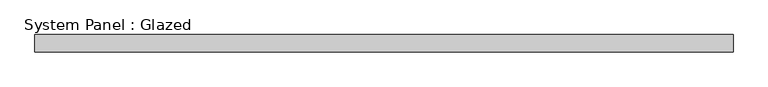
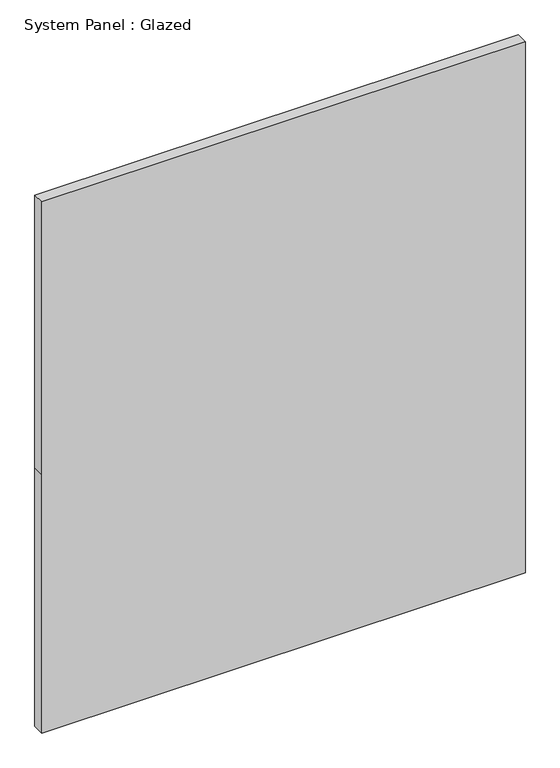
"""IFC4 building model written with IfcOpenShell, lengths in millimetres: plate geometry, System Panel : Glazed."""

import ifcopenshell
import ifcopenshell.guid

model = None  # the IFC model being written
_history = None  # IfcOwnerHistory: only IFC2X3 demands one
_inside = {}  # id of a spatial element -> (the spatial element, [elements in it])
_under = {}  # id of a project, library or spatial element -> (it, [spatial elements below it])
_declared = {}  # id of a project -> (the project, [libraries it declares])
_typed = {}  # id of a type object -> (the type object, [elements of that type])
_made_of = {}  # id of a material, layer set ... -> (it, [elements and type objects made of it])


def new_model(schema):
    """Start an empty IFC model of exactly this schema.

    Asked for "IFC4X3", IfcOpenShell would pick the latest addendum, in which some entities
    have other attributes; the version numbers below select the first issue.
    IFC2X3 requires an IfcOwnerHistory on every rooted entity: one is made here for all.
    """
    global model, _history
    if schema == "IFC4X3":
        model = ifcopenshell.file(schema_version=(4, 3, 0, 0))
    else:
        model = ifcopenshell.file(schema=schema)
    _inside.clear()
    _under.clear()
    _declared.clear()
    _typed.clear()
    _made_of.clear()
    _history = None
    if model.schema == "IFC2X3":
        org = make("IfcOrganization", Name="unknown")
        user = make(
            "IfcPersonAndOrganization",
            ThePerson=make("IfcPerson", FamilyName="unknown"),
            TheOrganization=org,
        )
        app = make(
            "IfcApplication",
            ApplicationDeveloper=org,
            Version="unknown",
            ApplicationFullName="unknown",
            ApplicationIdentifier="unknown",
        )
        _history = make(
            "IfcOwnerHistory",
            OwningUser=user,
            OwningApplication=app,
            ChangeAction="ADDED",
            CreationDate=0,
        )
    return model


def make(cls, **values):
    """One entity of the class cls with the attributes given. An attribute that is None is left unset."""
    return model.create_entity(
        cls, **{name: value for name, value in values.items() if value is not None}
    )


def rooted(cls, **values):
    """An entity with a GlobalId (a new one), such as an element, a storey or a relation."""
    return make(cls, GlobalId=ifcopenshell.guid.new(), OwnerHistory=_history, **values)


def si_unit(unit_type, name, prefix=None):
    """IfcSIUnit, for example si_unit("LENGTHUNIT", "METRE", prefix="MILLI")."""
    return make("IfcSIUnit", UnitType=unit_type, Prefix=prefix, Name=name)


def assignment(units):
    """IfcUnitAssignment: the units of a project."""
    return None if units is None else make("IfcUnitAssignment", Units=units)


def point(xyz):
    """IfcCartesianPoint."""
    return None if xyz is None else make("IfcCartesianPoint", Coordinates=xyz)


def direction(xyz):
    """IfcDirection."""
    return None if xyz is None else make("IfcDirection", DirectionRatios=xyz)


def frame(location, z_axis=None, x_axis=None):
    """IfcAxis2Placement3D, a coordinate frame: its origin and axes. An axis left out is left unset."""
    return make(
        "IfcAxis2Placement3D",
        Location=point(location),
        Axis=direction(z_axis),
        RefDirection=direction(x_axis),
    )


def origin():
    """The frame at (0, 0, 0) with its axes left unset."""
    return frame((0.0, 0.0, 0.0))


def place(relative_to, where):
    """IfcLocalPlacement: puts the frame where relative to a parent placement (None: the world)."""
    return make(
        "IfcLocalPlacement", PlacementRelTo=relative_to, RelativePlacement=where
    )


def context(
    kind, dimensions, precision=None, world=None, true_north=None, identifier=None
):
    """IfcGeometricRepresentationContext, for example the 3D "Model" context."""
    return make(
        "IfcGeometricRepresentationContext",
        ContextIdentifier=identifier,
        ContextType=kind,
        CoordinateSpaceDimension=dimensions,
        Precision=precision,
        WorldCoordinateSystem=world,
        TrueNorth=true_north,
    )


def project(units=None, contexts=None):
    """IfcProject with its units and contexts."""
    return rooted(
        "IfcProject",
        Name="project",
        RepresentationContexts=contexts,
        UnitsInContext=assignment(units),
    )


def spatial(cls, under=None, at=None, **own):
    """A site, building, storey or space (cls), placed at a placement, below another one or the project."""
    s = rooted(cls, ObjectPlacement=at, **own)
    if under is not None:
        _under.setdefault(under.id(), (under, []))[1].append(s)
    return s


def polyline(points):
    """IfcPolyline through the points."""
    return make("IfcPolyline", Points=[point(p) for p in points])


def outline(outer, holes=None, kind="AREA"):
    """IfcArbitraryClosedProfileDef: a profile drawn as a closed curve; with holes, ...WithVoids."""
    if holes is None:
        return make("IfcArbitraryClosedProfileDef", ProfileType=kind, OuterCurve=outer)
    return make(
        "IfcArbitraryProfileDefWithVoids",
        ProfileType=kind,
        OuterCurve=outer,
        InnerCurves=holes,
    )


def extrude(swept, where, along, depth):
    """IfcExtrudedAreaSolid: the profile swept, set in the frame where, extruded along a direction by depth."""
    return make(
        "IfcExtrudedAreaSolid",
        SweptArea=swept,
        Position=where,
        ExtrudedDirection=direction(along),
        Depth=depth,
    )


def shape(context_of_items, identifier, shape_type, items):
    """IfcShapeRepresentation: the items that make up one representation, for example the "Body"."""
    return make(
        "IfcShapeRepresentation",
        ContextOfItems=context_of_items,
        RepresentationIdentifier=identifier,
        RepresentationType=shape_type,
        Items=items,
    )


def source(mapping_origin, context_of_items, identifier, shape_type, items):
    """IfcRepresentationMap: a shape defined once, which mapped items show again and again."""
    return make(
        "IfcRepresentationMap",
        MappingOrigin=mapping_origin,
        MappedRepresentation=shape(context_of_items, identifier, shape_type, items),
    )


def transform(
    local_origin,
    x_axis=None,
    y_axis=None,
    z_axis=None,
    scale=None,
    scale2=None,
    scale3=None,
    uniform=True,
):
    """IfcCartesianTransformationOperator3D, or its non-uniform kind. x_axis, y_axis, z_axis: its Axis1, 2, 3."""
    if uniform:
        return make(
            "IfcCartesianTransformationOperator3D",
            Axis1=direction(x_axis),
            Axis2=direction(y_axis),
            LocalOrigin=point(local_origin),
            Scale=scale,
            Axis3=direction(z_axis),
        )
    return make(
        "IfcCartesianTransformationOperator3DnonUniform",
        Axis1=direction(x_axis),
        Axis2=direction(y_axis),
        LocalOrigin=point(local_origin),
        Scale=scale,
        Axis3=direction(z_axis),
        Scale2=scale2,
        Scale3=scale3,
    )


def mapped(mapping_source, mapping_target):
    """IfcMappedItem: shows the shape of a source again, moved by a transform."""
    return make(
        "IfcMappedItem", MappingSource=mapping_source, MappingTarget=mapping_target
    )


def made_of(thing, what):
    """Note that an element or type object is made of a material, layer set ...; save() writes the relation."""
    if what is not None:
        _made_of.setdefault(what.id(), (what, []))[1].append(thing)
    return thing


def element(
    cls,
    number,
    at=None,
    inside=None,
    cuts=None,
    type_object=None,
    material=None,
    context=None,
    identifier="Body",
    shape_type=None,
    held_by="IfcProductDefinitionShape",
    body=None,
    shapes=None,
    **own,
):
    """One element of the class cls, such as IfcWall. Its Tag is "e" and its number.

    at: its placement. inside: the storey or other place that contains it. cuts: it is an
    opening in that element (IfcRelVoidsElement). A single representation is given by context,
    identifier, shape_type and body (its items); several are given by shapes. held_by: the class
    of the entity that holds the representations. save() writes the other relations.
    """
    e = rooted(cls, Tag="e%d" % number, ObjectPlacement=at, **own)
    if body is not None:
        shapes = [shape(context, identifier, shape_type, body)]
    if shapes is not None:
        e.Representation = make(held_by, Representations=shapes)
    if inside is not None:
        _inside.setdefault(inside.id(), (inside, []))[1].append(e)
    if cuts is not None:
        rooted(
            "IfcRelVoidsElement", RelatingBuildingElement=cuts, RelatedOpeningElement=e
        )
    if type_object is not None:
        _typed.setdefault(type_object.id(), (type_object, []))[1].append(e)
    return made_of(e, material)


def aggregate(whole, parts):
    """IfcRelAggregates: a whole, such as a stair, and the parts it consists of."""
    return rooted("IfcRelAggregates", RelatingObject=whole, RelatedObjects=parts)


def save(model, path):
    """Write the relations noted so far, then the file.

    IfcRelAggregates (storeys below a building ...), IfcRelContainedInSpatialStructure (elements
    in a storey), IfcRelDefinesByType, IfcRelAssociatesMaterial and IfcRelDeclares: one each for
    every whole, place, type object, material and project.
    """
    for whole, parts in _under.values():
        aggregate(whole, parts)
    for where, things in _inside.values():
        rooted(
            "IfcRelContainedInSpatialStructure",
            RelatedElements=things,
            RelatingStructure=where,
        )
    for kind, things in _typed.values():
        rooted("IfcRelDefinesByType", RelatedObjects=things, RelatingType=kind)
    for what, things in _made_of.values():
        rooted("IfcRelAssociatesMaterial", RelatedObjects=things, RelatingMaterial=what)
    for by, libraries in _declared.values():
        rooted("IfcRelDeclares", RelatingContext=by, RelatedDefinitions=libraries)
    model.write(path)


def system_panel_glazed_21040209(model_context):
    return source(origin(), model_context, "Body", "SweptSolid", [
        extrude(outline(polyline([(0.0, -511.4925), (0.0, 511.4925), (577.85, 511.4925), (1187.45, 511.4925), (1187.45, -511.4925), (577.85, -511.4925), (0.0, -511.4925)])), frame((0.0, -44.45, 0.0), z_axis=(0.0, 1.0, 0.0), x_axis=(0.0, 0.0, 1.0)), (0.0, 0.0, 1.0), 25.4),
    ])


if __name__ == "__main__":
    model = new_model("IFC4")
    model_context = context("Model", 3, world=origin())
    ifc_project = project(units=[si_unit("LENGTHUNIT", "METRE", prefix="MILLI")], contexts=[model_context])
    site = spatial("IfcSite", under=ifc_project)
    building = spatial("IfcBuilding", under=site)
    placement = place(None, origin())
    system_panel_glazed_shape = system_panel_glazed_21040209(model_context)
    element("IfcPlate", 1, ObjectType="System Panel : Glazed", at=placement, inside=building, context=model_context, shape_type="MappedRepresentation", body=[
        mapped(system_panel_glazed_shape, transform((0.0, 0.0, 0.0), x_axis=(1.0, 0.0, 0.0), y_axis=(0.0, 1.0, 0.0), z_axis=(0.0, 0.0, 1.0))),
    ])
    save(model, "model.ifc")

# Revit data of these elements
# Project information
#   SR Document GUID = "7e8cea01-ee78-400c-8c48-bf15b658b500"
# Element 1 (IfcPlate, "System Panel : Glazed")
#   Materials on its faces: "Glass"
# Materials
#   "Glass": class "Unassigned", colour RGB 0 0 255, transparency 0.75
